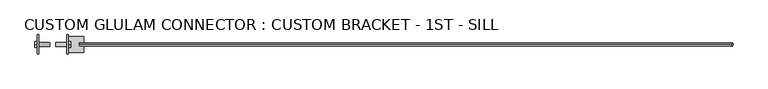
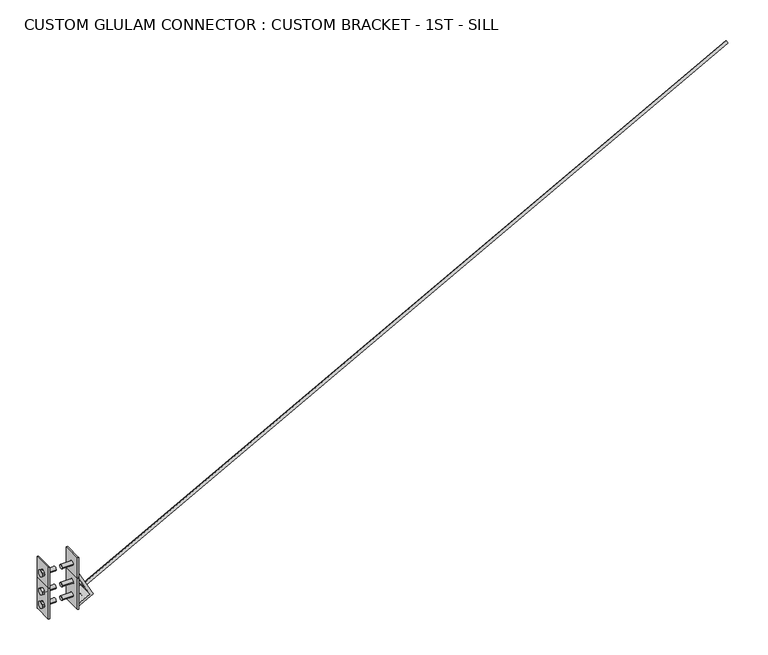
"""IFC4 building model written with IfcOpenShell, lengths in millimetres: fastener geometry, CUSTOM GLULAM CONNECTOR : CUSTOM BRACKET - 1ST - SILL."""

from ifc_helpers import new_model, si_unit, point, frame, frame_2d, origin, place, context, project, spatial, polyline, circle_curve, trimmed, segment, composite_curve, outline, extrude, source, transform, mapped, element, save
from ifc_brep_helpers import plane_surface, revolved_surface, advanced_brep


def custom_glulam_connector_custom_bracket_1st_sill_b9bb6f32(model_context):
    return source(origin(), model_context, "Body", "SolidModel", [
        advanced_brep(
        [(-87.3125, -13.890625, 160.3375), (-87.3125, 13.890625, 160.3375), (-95.25, 13.890625, 160.3375), (-95.25, -13.890625, 160.3375), (-95.25, 60.325, 211.1375), (-95.25, 60.325, 7.9375), (-95.25, 52.3875, 7.9375), (-95.25, -60.325, 7.9375), (-95.25, -60.325, 211.1375), (-95.25, 52.3875, 211.1375), (-95.25, 13.890625, 71.4375), (-95.25, -13.890625, 71.4375), (-87.3125, 13.890625, 71.4375), (-87.3125, -13.890625, 71.4375), (-87.3125, 60.325, 211.1375), (-87.3125, -60.325, 211.1375), (-87.3125, -60.325, 7.9375), (-87.3125, 60.325, 7.9375)],
        [
            (0, 1, circle_curve(frame((-87.3125, 0.0, 160.3375), z_axis=(1.0, 0.0, 0.0), x_axis=(0.0, 1.0, 0.0)), 13.890625)),
            (1, 2),
            (2, 3, circle_curve(frame((-95.25, 0.0, 160.3375), z_axis=(-1.0, 0.0, 0.0), x_axis=(0.0, 1.0, 0.0)), 13.890625)),
            (3, 0),
            (4, 5),
            (5, 6),
            (6, 7),
            (7, 8),
            (8, 9),
            (9, 4),
            (10, 11, circle_curve(frame((-95.25, 0.0, 71.4375), z_axis=(1.0, 0.0, 0.0), x_axis=(0.0, 1.0, 0.0)), 13.890625)),
            (11, 10, circle_curve(frame((-95.25, 0.0, 71.4375), z_axis=(1.0, 0.0, 0.0), x_axis=(0.0, 1.0, 0.0)), 13.890625)),
            (2, 3, circle_curve(frame((-95.25, 0.0, 160.3375), z_axis=(1.0, 0.0, 0.0), x_axis=(0.0, 1.0, 0.0)), 13.890625)),
            (10, 12),
            (12, 13, circle_curve(frame((-87.3125, 0.0, 71.4375), z_axis=(1.0, 0.0, 0.0), x_axis=(0.0, 1.0, 0.0)), 13.890625)),
            (13, 11),
            (1, 0, circle_curve(frame((-87.3125, 0.0, 160.3375), z_axis=(1.0, 0.0, 0.0), x_axis=(0.0, 1.0, 0.0)), 13.890625)),
            (13, 12, circle_curve(frame((-87.3125, 0.0, 71.4375), z_axis=(1.0, 0.0, 0.0), x_axis=(0.0, 1.0, 0.0)), 13.890625)),
            (14, 15),
            (15, 16),
            (16, 17),
            (17, 14),
            (8, 15),
            (14, 4),
            (7, 16),
            (5, 17),
        ],
        [
            revolved_surface(polyline([(-95.25, 13.890625, 160.3375), (-87.3125, 13.890625, 160.3375)]), (-87.3125, 0.0, 160.3375), (-1.0, 0.0, 0.0)),
            plane_surface(frame((-95.25, -60.325, 211.1375), z_axis=(-1.0, 0.0, 0.0), x_axis=(0.0, -1.0, 0.0))),
            revolved_surface(polyline([(-95.25, 13.890625, 71.4375), (-87.3125, 13.890625, 71.4375)]), (-87.3125, 0.0, 71.4375), (-1.0, 0.0, 0.0)),
            plane_surface(frame((-87.3125, -60.325, 211.1375), z_axis=(1.0, 0.0, 0.0), x_axis=(0.0, 1.0, 0.0))),
            plane_surface(frame((-95.25, 60.325, 211.1375), z_axis=(0.0, 0.0, 1.0), x_axis=(1.0, 0.0, 0.0))),
            plane_surface(frame((-95.25, -60.325, 211.1375), z_axis=(0.0, -1.0, 0.0), x_axis=(1.0, 0.0, 0.0))),
            plane_surface(frame((-95.25, -60.325, 7.9375), z_axis=(0.0, 0.0, -1.0), x_axis=(1.0, 0.0, 0.0))),
            plane_surface(frame((-95.25, 60.325, 7.9375), z_axis=(0.0, 1.0, 0.0), x_axis=(1.0, 0.0, 0.0))),
        ],
        [
            (0, [[1, 2, 3, 4]]),
            (1, [[5, 6, 7, 8, 9, 10], [11, 12], [13, -3]]),
            (2, [[-11, 14, 15, 16]]),
            (0, [[-13, -2, 17, -4]]),
            (2, [[18, -14, -12, -16]]),
            (3, [[19, 20, 21, 22], [-17, -1], [-15, -18]]),
            (4, [[23, -19, 24, -10, -9]]),
            (5, [[25, -20, -23, -8]]),
            (6, [[26, -21, -25, -7, -6]]),
            (7, [[-24, -22, -26, -5]]),
        ],
    ),
        extrude(outline(polyline([(-19.05, 171.3360226), (0.0, 182.3345453), (19.05, 171.3360226), (19.05, 149.3389774), (0.0, 138.3404547), (-19.05, 149.3389774), (-19.05, 171.3360226)])), frame((-110.2320312, 0.0, 0.0), z_axis=(1.0, 0.0, 0.0), x_axis=(0.0, 1.0, 0.0)), (0.0, 0.0, 1.0), 14.9820312),
        extrude(outline(composite_curve([segment(trimmed(circle_curve(frame_2d((0.0, 160.3375)), 12.7), [point((-12.7, 160.3375))], [point((12.7, 160.3375))], False, "CARTESIAN"), True, "CONTINUOUS"), segment(trimmed(circle_curve(frame_2d((0.0, 160.3375)), 12.7), [point((12.7, 160.3375))], [point((-12.7, 160.3375))], False, "CARTESIAN"), True, "CONTINUOUS")], self_intersect=False)), frame((-95.25, 0.0, 0.0), z_axis=(1.0, 0.0, 0.0), x_axis=(0.0, 1.0, 0.0)), (0.0, 0.0, 1.0), 76.2),
        extrude(outline(polyline([(-19.05, 82.4360226), (0.0, 93.4345453), (19.05, 82.4360226), (19.05, 60.4389774), (0.0, 49.4404547), (-19.05, 60.4389774), (-19.05, 82.4360226)])), frame((-110.2320312, 0.0, 0.0), z_axis=(1.0, 0.0, 0.0), x_axis=(0.0, 1.0, 0.0)), (0.0, 0.0, 1.0), 14.9820312),
        extrude(outline(composite_curve([segment(trimmed(circle_curve(frame_2d((0.0, 71.4375)), 12.7), [point((-12.7, 71.4375))], [point((12.7, 71.4375))], False, "CARTESIAN"), True, "CONTINUOUS"), segment(trimmed(circle_curve(frame_2d((0.0, 71.4375)), 12.7), [point((12.7, 71.4375))], [point((-12.7, 71.4375))], False, "CARTESIAN"), True, "CONTINUOUS")], self_intersect=False)), frame((-95.25, 0.0, 0.0), z_axis=(1.0, 0.0, 0.0), x_axis=(0.0, 1.0, 0.0)), (0.0, 0.0, 1.0), 76.2),
        extrude(outline(polyline([(-19.05, 171.3360226), (0.0, 182.3345453), (19.05, 171.3360226), (19.05, 149.3389774), (0.0, 138.3404547), (-19.05, 149.3389774), (-19.05, 171.3360226)])), frame((-110.2320312, 0.0, 0.0), z_axis=(1.0, 0.0, 0.0), x_axis=(0.0, 1.0, 0.0)), (0.0, 0.0, 1.0), 14.9820312),
        extrude(outline(composite_curve([segment(trimmed(circle_curve(frame_2d((0.0, 160.3375)), 12.7), [point((-12.7, 160.3375))], [point((12.7, 160.3375))], False, "CARTESIAN"), True, "CONTINUOUS"), segment(trimmed(circle_curve(frame_2d((0.0, 160.3375)), 12.7), [point((12.7, 160.3375))], [point((-12.7, 160.3375))], False, "CARTESIAN"), True, "CONTINUOUS")], self_intersect=False)), frame((-95.25, 0.0, 0.0), z_axis=(1.0, 0.0, 0.0), x_axis=(0.0, 1.0, 0.0)), (0.0, 0.0, 1.0), 76.2),
        extrude(outline(polyline([(-19.05, 171.3360226), (0.0, 182.3345453), (19.05, 171.3360226), (19.05, 149.3389774), (0.0, 138.3404547), (-19.05, 149.3389774), (-19.05, 171.3360226)])), frame((95.25, 0.0, 0.0), z_axis=(1.0, 0.0, 0.0), x_axis=(0.0, 1.0, 0.0)), (0.0, 0.0, 1.0), 14.9820312),
        extrude(outline(composite_curve([segment(trimmed(circle_curve(frame_2d((0.0, 160.3375)), 12.7), [point((-12.7, 160.3375))], [point((12.7, 160.3375))], False, "CARTESIAN"), True, "CONTINUOUS"), segment(trimmed(circle_curve(frame_2d((0.0, 160.3375)), 12.7), [point((12.7, 160.3375))], [point((-12.7, 160.3375))], False, "CARTESIAN"), True, "CONTINUOUS")], self_intersect=False)), frame((19.05, 0.0, 0.0), z_axis=(1.0, 0.0, 0.0), x_axis=(0.0, 1.0, 0.0)), (0.0, 0.0, 1.0), 76.2),
        extrude(outline(polyline([(-19.05, 82.4360226), (0.0, 93.4345453), (19.05, 82.4360226), (19.05, 60.4389774), (0.0, 49.4404547), (-19.05, 60.4389774), (-19.05, 82.4360226)])), frame((95.25, 0.0, 0.0), z_axis=(1.0, 0.0, 0.0), x_axis=(0.0, 1.0, 0.0)), (0.0, 0.0, 1.0), 14.9820312),
        extrude(outline(composite_curve([segment(trimmed(circle_curve(frame_2d((0.0, 71.4375)), 12.7), [point((-12.7, 71.4375))], [point((12.7, 71.4375))], False, "CARTESIAN"), True, "CONTINUOUS"), segment(trimmed(circle_curve(frame_2d((0.0, 71.4375)), 12.7), [point((12.7, 71.4375))], [point((-12.7, 71.4375))], False, "CARTESIAN"), True, "CONTINUOUS")], self_intersect=False)), frame((19.05, 0.0, 0.0), z_axis=(1.0, 0.0, 0.0), x_axis=(0.0, 1.0, 0.0)), (0.0, 0.0, 1.0), 76.2),
        extrude(outline(polyline([(-19.05, 171.3360226), (0.0, 182.3345453), (19.05, 171.3360226), (19.05, 149.3389774), (0.0, 138.3404547), (-19.05, 149.3389774), (-19.05, 171.3360226)])), frame((95.25, 0.0, 0.0), z_axis=(1.0, 0.0, 0.0), x_axis=(0.0, 1.0, 0.0)), (0.0, 0.0, 1.0), 14.9820312),
        extrude(outline(composite_curve([segment(trimmed(circle_curve(frame_2d((0.0, 160.3375)), 12.7), [point((-12.7, 160.3375))], [point((12.7, 160.3375))], False, "CARTESIAN"), True, "CONTINUOUS"), segment(trimmed(circle_curve(frame_2d((0.0, 160.3375)), 12.7), [point((12.7, 160.3375))], [point((-12.7, 160.3375))], False, "CARTESIAN"), True, "CONTINUOUS")], self_intersect=False)), frame((19.05, 0.0, 0.0), z_axis=(1.0, 0.0, 0.0), x_axis=(0.0, 1.0, 0.0)), (0.0, 0.0, 1.0), 76.2),
        advanced_brep(
        [(87.3125, -13.890625, 160.3375), (95.25, -13.890625, 160.3375), (95.25, 13.890625, 160.3375), (87.3125, 13.890625, 160.3375), (95.25, 60.325, 211.1375), (95.25, 52.3875, 211.1375), (95.25, -60.325, 211.1375), (95.25, -60.325, 7.9375), (95.25, 52.3875, 7.9375), (95.25, 60.325, 7.9375), (95.25, 13.890625, 71.4375), (95.25, -13.890625, 71.4375), (87.3125, -13.890625, 71.4375), (87.3125, 13.890625, 71.4375), (87.3125, 60.325, 211.1375), (87.3125, 60.325, 7.9375), (87.3125, -60.325, 7.9375), (87.3125, -60.325, 211.1375)],
        [
            (0, 1),
            (1, 2, circle_curve(frame((95.25, 0.0, 160.3375), z_axis=(1.0, 0.0, 0.0), x_axis=(0.0, 1.0, 0.0)), 13.890625)),
            (2, 3),
            (3, 0, circle_curve(frame((87.3125, 0.0, 160.3375), z_axis=(-1.0, 0.0, 0.0), x_axis=(0.0, 1.0, 0.0)), 13.890625)),
            (4, 5),
            (5, 6),
            (6, 7),
            (7, 8),
            (8, 9),
            (9, 4),
            (1, 2, circle_curve(frame((95.25, 0.0, 160.3375), z_axis=(-1.0, 0.0, 0.0), x_axis=(0.0, 1.0, 0.0)), 13.890625)),
            (10, 11, circle_curve(frame((95.25, 0.0, 71.4375), z_axis=(-1.0, 0.0, 0.0), x_axis=(0.0, 1.0, 0.0)), 13.890625)),
            (11, 10, circle_curve(frame((95.25, 0.0, 71.4375), z_axis=(-1.0, 0.0, 0.0), x_axis=(0.0, 1.0, 0.0)), 13.890625)),
            (11, 12),
            (12, 13, circle_curve(frame((87.3125, 0.0, 71.4375), z_axis=(-1.0, 0.0, 0.0), x_axis=(0.0, 1.0, 0.0)), 13.890625)),
            (13, 10),
            (0, 3, circle_curve(frame((87.3125, 0.0, 160.3375), z_axis=(-1.0, 0.0, 0.0), x_axis=(0.0, 1.0, 0.0)), 13.890625)),
            (13, 12, circle_curve(frame((87.3125, 0.0, 71.4375), z_axis=(-1.0, 0.0, 0.0), x_axis=(0.0, 1.0, 0.0)), 13.890625)),
            (14, 15),
            (15, 16),
            (16, 17),
            (17, 14),
            (4, 14),
            (17, 6),
            (16, 7),
            (15, 9),
        ],
        [
            revolved_surface(polyline([(95.25, 13.890625, 160.3375), (87.3125, 13.890625, 160.3375)]), (87.3125, 0.0, 160.3375), (1.0, 0.0, 0.0)),
            plane_surface(frame((95.25, -60.325, 211.1375), z_axis=(1.0, 0.0, 0.0), x_axis=(0.0, -1.0, 0.0))),
            revolved_surface(polyline([(95.25, 13.890625, 71.4375), (87.3125, 13.890625, 71.4375)]), (87.3125, 0.0, 71.4375), (1.0, 0.0, 0.0)),
            plane_surface(frame((87.3125, -60.325, 211.1375), z_axis=(-1.0, 0.0, 0.0), x_axis=(0.0, 1.0, 0.0))),
            plane_surface(frame((95.25, 60.325, 211.1375), z_axis=(0.0, 0.0, 1.0), x_axis=(-1.0, 0.0, 0.0))),
            plane_surface(frame((95.25, -60.325, 211.1375), z_axis=(0.0, -1.0, 0.0), x_axis=(-1.0, 0.0, 0.0))),
            plane_surface(frame((95.25, -60.325, 7.9375), z_axis=(0.0, 0.0, -1.0), x_axis=(-1.0, 0.0, 0.0))),
            plane_surface(frame((95.25, 60.325, 7.9375), z_axis=(0.0, 1.0, 0.0), x_axis=(-1.0, 0.0, 0.0))),
        ],
        [
            (0, [[1, 2, 3, 4]]),
            (1, [[5, 6, 7, 8, 9, 10], [-2, 11], [12, 13]]),
            (2, [[14, 15, 16, -13]]),
            (0, [[-1, 17, -3, -11]]),
            (2, [[-14, -12, -16, 18]]),
            (3, [[19, 20, 21, 22], [-4, -17], [-18, -15]]),
            (4, [[-6, -5, 23, -22, 24]]),
            (5, [[-7, -24, -21, 25]]),
            (6, [[-9, -8, -25, -20, 26]]),
            (7, [[-10, -26, -19, -23]]),
        ],
    ),
        extrude(outline(polyline([(-19.05, 291.9860226), (0.0, 302.9845453), (19.05, 291.9860226), (19.05, 269.9889774), (0.0, 258.9904547), (-19.05, 269.9889774), (-19.05, 291.9860226)])), frame((-110.2320312, 0.0, 0.0), z_axis=(1.0, 0.0, 0.0), x_axis=(0.0, 1.0, 0.0)), (0.0, 0.0, 1.0), 14.9820312),
        extrude(outline(composite_curve([segment(trimmed(circle_curve(frame_2d((0.0, 280.9875)), 12.7), [point((-12.7, 280.9875))], [point((12.7, 280.9875))], False, "CARTESIAN"), True, "CONTINUOUS"), segment(trimmed(circle_curve(frame_2d((0.0, 280.9875)), 12.7), [point((12.7, 280.9875))], [point((-12.7, 280.9875))], False, "CARTESIAN"), True, "CONTINUOUS")], self_intersect=False)), frame((-95.25, 0.0, 0.0), z_axis=(1.0, 0.0, 0.0), x_axis=(0.0, 1.0, 0.0)), (0.0, 0.0, 1.0), 76.2),
        advanced_brep(
        [(-95.25, 60.325, 350.8375), (-87.3125, 60.325, 350.8375), (-87.3125, 60.325, 211.1375), (-95.25, 60.325, 211.1375), (-87.3125, -13.890625, 280.9875), (-87.3125, 13.890625, 280.9875), (-95.25, 13.890625, 280.9875), (-95.25, -13.890625, 280.9875), (-95.25, -60.325, 350.8375), (-87.3125, -60.325, 350.8375), (-95.25, -52.3875, 350.8375), (-95.25, -52.3875, 211.1375), (-95.25, -60.325, 211.1375), (-87.3125, -60.325, 211.1375)],
        [
            (0, 1),
            (1, 2),
            (2, 3),
            (3, 0),
            (4, 5, circle_curve(frame((-87.3125, 0.0, 280.9875), z_axis=(1.0, 0.0, 0.0), x_axis=(0.0, 1.0, 0.0)), 13.890625)),
            (5, 6),
            (6, 7, circle_curve(frame((-95.25, 0.0, 280.9875), z_axis=(-1.0, 0.0, 0.0), x_axis=(0.0, 1.0, 0.0)), 13.890625)),
            (7, 4),
            (7, 6, circle_curve(frame((-95.25, 0.0, 280.9875), z_axis=(-1.0, 0.0, 0.0), x_axis=(0.0, 1.0, 0.0)), 13.890625)),
            (5, 4, circle_curve(frame((-87.3125, 0.0, 280.9875), z_axis=(1.0, 0.0, 0.0), x_axis=(0.0, 1.0, 0.0)), 13.890625)),
            (8, 9),
            (9, 1),
            (0, 10),
            (10, 8),
            (3, 11),
            (11, 12),
            (12, 8),
            (9, 13),
            (13, 2),
            (12, 13),
        ],
        [
            plane_surface(frame((-95.25, 60.325, 211.1375), z_axis=(0.0, 1.0, 0.0), x_axis=(1.0, 0.0, 0.0))),
            revolved_surface(polyline([(-95.25, 13.890625, 280.9875), (-87.3125, 13.890625, 280.9875)]), (-87.3125, 0.0, 280.9875), (-1.0, 0.0, 0.0)),
            plane_surface(frame((-95.25, 60.325, 350.8375), z_axis=(0.0, 0.0, 1.0), x_axis=(1.0, 0.0, 0.0))),
            plane_surface(frame((-95.25, -60.325, 350.8375), z_axis=(-1.0, 0.0, 0.0), x_axis=(0.0, -1.0, 0.0))),
            plane_surface(frame((-87.3125, -60.325, 350.8375), z_axis=(1.0, 0.0, 0.0), x_axis=(0.0, 1.0, 0.0))),
            plane_surface(frame((-95.25, -60.325, 350.8375), z_axis=(0.0, -1.0, 0.0), x_axis=(1.0, 0.0, 0.0))),
            plane_surface(frame((-95.25, -60.325, 211.1375), z_axis=(0.0, 0.0, -1.0), x_axis=(1.0, 0.0, 0.0))),
        ],
        [
            (0, [[1, 2, 3, 4]]),
            (1, [[5, 6, 7, 8]]),
            (1, [[9, -6, 10, -8]]),
            (2, [[11, 12, -1, 13, 14]]),
            (3, [[-4, 15, 16, 17, -14, -13], [-9, -7]]),
            (4, [[-12, 18, 19, -2], [-10, -5]]),
            (5, [[20, -18, -11, -17]]),
            (6, [[-3, -19, -20, -16, -15]]),
        ],
    ),
        advanced_brep(
        [(95.25, 60.325, 350.8375), (95.25, 60.325, 211.1375), (87.3125, 60.325, 211.1375), (87.3125, 60.325, 350.8375), (87.3125, -13.890625, 280.9875), (95.25, -13.890625, 280.9875), (95.25, 13.890625, 280.9875), (87.3125, 13.890625, 280.9875), (95.25, -60.325, 350.8375), (95.25, -52.3875, 350.8375), (87.3125, -60.325, 350.8375), (95.25, -60.325, 211.1375), (95.25, -52.3875, 211.1375), (87.3125, -60.325, 211.1375)],
        [
            (0, 1),
            (1, 2),
            (2, 3),
            (3, 0),
            (4, 5),
            (5, 6, circle_curve(frame((95.25, 0.0, 280.9875), z_axis=(1.0, 0.0, 0.0), x_axis=(0.0, 1.0, 0.0)), 13.890625)),
            (6, 7),
            (7, 4, circle_curve(frame((87.3125, 0.0, 280.9875), z_axis=(-1.0, 0.0, 0.0), x_axis=(0.0, 1.0, 0.0)), 13.890625)),
            (4, 7, circle_curve(frame((87.3125, 0.0, 280.9875), z_axis=(-1.0, 0.0, 0.0), x_axis=(0.0, 1.0, 0.0)), 13.890625)),
            (6, 5, circle_curve(frame((95.25, 0.0, 280.9875), z_axis=(1.0, 0.0, 0.0), x_axis=(0.0, 1.0, 0.0)), 13.890625)),
            (8, 9),
            (9, 0),
            (3, 10),
            (10, 8),
            (8, 11),
            (11, 12),
            (12, 1),
            (2, 13),
            (13, 10),
            (13, 11),
        ],
        [
            plane_surface(frame((95.25, 60.325, 211.1375), z_axis=(0.0, 1.0, 0.0), x_axis=(-1.0, 0.0, 0.0))),
            revolved_surface(polyline([(95.25, 13.890625, 280.9875), (87.3125, 13.890625, 280.9875)]), (87.3125, 0.0, 280.9875), (1.0, 0.0, 0.0)),
            plane_surface(frame((95.25, 60.325, 350.8375), z_axis=(0.0, 0.0, 1.0), x_axis=(-1.0, 0.0, 0.0))),
            plane_surface(frame((95.25, -60.325, 350.8375), z_axis=(1.0, 0.0, 0.0), x_axis=(0.0, -1.0, 0.0))),
            plane_surface(frame((87.3125, -60.325, 350.8375), z_axis=(-1.0, 0.0, 0.0), x_axis=(0.0, 1.0, 0.0))),
            plane_surface(frame((95.25, -60.325, 350.8375), z_axis=(0.0, -1.0, 0.0), x_axis=(-1.0, 0.0, 0.0))),
            plane_surface(frame((95.25, -60.325, 211.1375), z_axis=(0.0, 0.0, -1.0), x_axis=(-1.0, 0.0, 0.0))),
        ],
        [
            (0, [[1, 2, 3, 4]]),
            (1, [[5, 6, 7, 8]]),
            (1, [[-5, 9, -7, 10]]),
            (2, [[11, 12, -4, 13, 14]]),
            (3, [[-12, -11, 15, 16, 17, -1], [-6, -10]]),
            (4, [[-3, 18, 19, -13], [-8, -9]]),
            (5, [[-15, -14, -19, 20]]),
            (6, [[-17, -16, -20, -18, -2]]),
        ],
    ),
        extrude(outline(polyline([(-19.05, 291.9860226), (0.0, 302.9845453), (19.05, 291.9860226), (19.05, 269.9889774), (0.0, 258.9904547), (-19.05, 269.9889774), (-19.05, 291.9860226)])), frame((95.25, 0.0, 0.0), z_axis=(1.0, 0.0, 0.0), x_axis=(0.0, 1.0, 0.0)), (0.0, 0.0, 1.0), 14.9820312),
        extrude(outline(composite_curve([segment(trimmed(circle_curve(frame_2d((0.0, 280.9875)), 12.7), [point((-12.7, 280.9875))], [point((12.7, 280.9875))], False, "CARTESIAN"), True, "CONTINUOUS"), segment(trimmed(circle_curve(frame_2d((0.0, 280.9875)), 12.7), [point((12.7, 280.9875))], [point((-12.7, 280.9875))], False, "CARTESIAN"), True, "CONTINUOUS")], self_intersect=False)), frame((19.05, 0.0, 0.0), z_axis=(1.0, 0.0, 0.0), x_axis=(0.0, 1.0, 0.0)), (0.0, 0.0, 1.0), 76.2),
        extrude(outline(composite_curve([segment(trimmed(circle_curve(frame_2d((0.0, -9.525)), 9.525), [point((0.0, -19.05))], [point((0.0, 0.0))], False, "CARTESIAN"), True, "CONTINUOUS"), segment(trimmed(circle_curve(frame_2d((0.0, -9.525)), 9.525), [point((0.0, 0.0))], [point((0.0, -19.05))], False, "CARTESIAN"), True, "CONTINUOUS")], self_intersect=False)), frame((173.2138238, 0.0, 105.1724436), z_axis=(0.8788171126619665, 0.0, 0.4771587602596065), x_axis=(0.0, -1.0, 0.0)), (0.0, 0.0, 1.0), 4597.4),
        advanced_brep(
        [(192.9085516, -50.8, 68.8992672), (95.25, -50.8, 248.7639444), (95.25, -50.8, 215.4940952), (171.3824347, -50.8, 75.2755936), (95.25, -50.8, 33.9390543), (95.25, -50.8, 15.875), (192.9085516, 50.8, 68.8992672), (95.25, 50.8, 15.875), (95.25, 50.8, 33.9390543), (171.3824347, 50.8, 75.2755936), (95.25, 50.8, 215.4940952), (95.25, 50.8, 248.7639444), (173.781941, 0.0, 104.1261019), (163.5558323, 0.0, 122.9602512), (149.6046106, 0.0, 115.3853559), (159.8307193, 0.0, 96.5512066), (141.0385275, 0.0, 58.8001963), (140.3409665, 0.0, 58.4214515), (147.9158618, 0.0, 44.4702298), (148.6134229, 0.0, 44.8489746)],
        [
            (0, 1),
            (1, 2),
            (2, 3),
            (3, 4),
            (4, 5),
            (5, 0),
            (6, 7),
            (7, 8),
            (8, 9),
            (9, 10),
            (10, 11),
            (11, 6),
            (0, 6),
            (11, 1),
            (12, 13, circle_curve(frame((168.6688866, 0.0, 113.5431766), z_axis=(-0.8788171126619665, 0.0, -0.4771587602596065), x_axis=(-0.4771587602596065, 0.0, 0.8788171126619665)), 10.715625)),
            (13, 12, circle_curve(frame((168.6688866, 0.0, 113.5431766), z_axis=(-0.8788171126619665, 0.0, -0.4771587602596065), x_axis=(-0.4771587602596065, 0.0, 0.8788171126619665)), 10.715625)),
            (10, 2),
            (9, 3),
            (14, 15, circle_curve(frame((154.717665, 0.0, 105.9682812), z_axis=(0.8788171126619665, 0.0, 0.4771587602596065), x_axis=(-0.4771587602596065, 0.0, 0.8788171126619665)), 10.715625)),
            (15, 14, circle_curve(frame((154.717665, 0.0, 105.9682812), z_axis=(0.8788171126619665, 0.0, 0.4771587602596065), x_axis=(-0.4771587602596065, 0.0, 0.8788171126619665)), 10.715625)),
            (8, 4),
            (16, 17, circle_curve(frame((140.689747, 0.0, 58.6108239), z_axis=(0.47715876025960524, 0.0, -0.8788171126619673), x_axis=(0.878817112661967, 0.0, 0.47715876025960513)), 0.396875)),
            (17, 16, circle_curve(frame((140.689747, 0.0, 58.6108239), z_axis=(0.47715876025960524, 0.0, -0.8788171126619673), x_axis=(0.878817112661967, 0.0, 0.47715876025960513)), 0.396875)),
            (7, 5),
            (18, 19, circle_curve(frame((148.2646423, 0.0, 44.6596022), z_axis=(-0.47715876025960524, 0.0, 0.8788171126619673), x_axis=(0.878817112661967, 0.0, 0.47715876025960513)), 0.396875)),
            (19, 18, circle_curve(frame((148.2646423, 0.0, 44.6596022), z_axis=(-0.47715876025960524, 0.0, 0.8788171126619673), x_axis=(0.878817112661967, 0.0, 0.47715876025960513)), 0.396875)),
            (12, 15),
            (14, 13),
            (18, 17),
            (16, 19),
        ],
        [
            plane_surface(frame((95.25, -50.8, 248.7639444), z_axis=(0.0, -1.0000000000000002, 0.0), x_axis=(-0.4771587602596065, 0.0, 0.8788171126619665))),
            plane_surface(frame((95.25, 50.8, 248.7639444), z_axis=(0.0, 1.0000000000000002, 0.0), x_axis=(0.4771587602596065, 0.0, -0.8788171126619665))),
            plane_surface(frame((192.9085516, -50.8, 68.8992672), z_axis=(0.8788171126619665, 0.0, 0.4771587602596065), x_axis=(0.0, 1.0, 0.0))),
            plane_surface(frame((95.25, -50.8, 248.7639444), z_axis=(-1.0, 0.0, 0.0), x_axis=(0.0, 1.0, 0.0))),
            plane_surface(frame((95.25, -50.8, 215.4940952), z_axis=(-0.8788171126619664, 0.0, -0.4771587602596066), x_axis=(0.0, 1.0, 0.0))),
            plane_surface(frame((171.3824347, -50.8, 75.2755936), z_axis=(-0.4771587602596049, 0.0, 0.8788171126619674), x_axis=(0.0, 1.0, 0.0))),
            plane_surface(frame((95.25, -50.8, 33.9390543), z_axis=(-1.0, 0.0, 0.0), x_axis=(0.0, 1.0, 0.0))),
            plane_surface(frame((95.25, -50.8, 15.875), z_axis=(0.4771587602596052, 0.0, -0.8788171126619672), x_axis=(0.0, 1.0, 0.0))),
            revolved_surface(polyline([(149.60461058960067, 0.0, 115.38535590022673), (163.55583228121063, 0.0, 122.9602512346057)]), (168.6688866, 0.0, 113.5431766), (-0.8788171126619665, 0.0, -0.4771587602596065)),
            revolved_surface(polyline([(141.0385274949113, 0.0, 58.80019629723707), (148.61342285819435, 0.0, 44.848974552392434)]), (148.2646423, 0.0, 44.6596022), (-0.47715876025960513, 0.0, 0.878817112661967)),
        ],
        [
            (0, [[1, 2, 3, 4, 5, 6]]),
            (1, [[7, 8, 9, 10, 11, 12]]),
            (2, [[-1, 13, -12, 14], [15, 16]]),
            (3, [[-2, -14, -11, 17]]),
            (4, [[-3, -17, -10, 18], [19, 20]]),
            (5, [[-4, -18, -9, 21], [22, 23]]),
            (6, [[-5, -21, -8, 24]]),
            (7, [[-6, -24, -7, -13], [25, 26]]),
            (8, [[27, -19, 28, -15]]),
            (8, [[-27, -16, -28, -20]]),
            (9, [[29, -22, 30, -25]]),
            (9, [[-29, -26, -30, -23]]),
        ],
    ),
    ])


if __name__ == "__main__":
    model = new_model("IFC4")
    model_context = context("Model", 3, world=origin())
    ifc_project = project(units=[si_unit("LENGTHUNIT", "METRE", prefix="MILLI")], contexts=[model_context])
    site = spatial("IfcSite", under=ifc_project)
    building = spatial("IfcBuilding", under=site)
    placement = place(None, origin())
    custom_glulam_connector_custom_bracket_1st_sill_shape = custom_glulam_connector_custom_bracket_1st_sill_b9bb6f32(model_context)
    element("IfcFastener", 1, ObjectType="CUSTOM GLULAM CONNECTOR : CUSTOM BRACKET - 1ST - SILL", at=placement, inside=building, context=model_context, shape_type="MappedRepresentation", body=[
        mapped(custom_glulam_connector_custom_bracket_1st_sill_shape, transform((0.0, 0.0, 0.0), x_axis=(1.0, 0.0, 0.0), y_axis=(0.0, 1.0, 0.0), z_axis=(0.0, 0.0, 1.0))),
    ])
    save(model, "model.ifc")

# Revit data of these elements
# Type "CUSTOM GLULAM CONNECTOR : CUSTOM BRACKET - 1ST - SILL"
#   Width - Top = 0' - 6 7/8"
#   Top/Bottom Plate Thickness = 0' - 0 5/16"
#   Top/Bottom Plate - Width = 0' - 7 1/2"
#   Rod Radius = 0' - 0 3/8"
#   Rod Length [instance default] = 1' - 0"
#   Plate Thickness = 0' - 0 5/16"
#   Offset - Upper Plate 2 = 0' - 0"
#   Height of Plate = 0' - 8"
#   Width - Bottom = 0' - 6 7/8"
#   Plate Width = 0' - 4 3/4"
#   Bracket Width = 0' - 4"
#   Bracket Thickness = 0' - 0 5/8"
#   Bracket Offset in X = 0' - 3 3/4"
#   Bracket Offset in Y = 0' - 0 3/8"
#   Bracket Offset = 0' - 0 5/8"
#   Bracket Leg = 0' - 4 3/8"
#   Bracket Hole Radius - Up = 0' - 0 27/64"
#   Bracket Hole Radius - Down = 0' - 0 1/64"
#   Bracket Hole Offset = 0' - 2"
#   Beam Width = 0' - 7 3/8"
#   Angle 2 = 28.50°
#   Angle 1 = 118.50°
#   Top Plate Visible = no
#   Rod Visibility = yes
#   Plate Visibility - Upper Right 2 = no
#   Plate Visibility - Upper Right 1 = yes
#   Plate Visibility - Upper Left 2 = no
#   Plate Visibility - Upper Left 1 = yes
#   Plate Visibility - Lower Right 2 = no
#   Plate Visibility - Lower Right 1 = yes
#   Plate Visibility - Lower Left 2 = no
#   Plate Visibility - Lower Left 1 = yes
#   Bracket Visibility = yes
#   Bottom Plate Visible = no
#   Upper Plates - 2 = element 1323965
#   Upper Plates - 1 = element 1323965
#   Lower Plates = element 1339837
#   Bracket Material = 5/8" STEEL ANGLE (HDG AFTER FABRICATION)
#   URL = ""
# Element 1 (IfcFastener, "CUSTOM GLULAM CONNECTOR : CUSTOM BRACKET - 1ST - SILL")
#   Rod Length = 15' - 1"
#   Materials on its faces: "1\" GALV. LAG BOLT (LENGTH = 1/2\" SHY OF GLULAM DEPTH) -  (GALV. THRU BOLT IF PLATE ON OPP. SIDE OF STRUCT MEMBER)", "5/16\" STEEL PLATE (HDG AFTER FABRICATION)", "5/8\" STEEL ANGLE (HDG AFTER FABRICATION)", "3/4\" GALV. ROD (THREADED AT ENDS) - TURN BUCKLE AT 1/4 POINT OF TOTAL LENGTH"
# Materials
#   "5/8\" STEEL ANGLE (HDG AFTER FABRICATION)": class "Generic", colour RGB 195 195 195, transparency 0, Cost = 0
#   "1\" GALV. LAG BOLT (LENGTH = 1/2\" SHY OF GLULAM DEPTH) -  (GALV. THRU BOLT IF PLATE ON OPP. SIDE OF STRUCT MEMBER)": class "Generic", colour RGB 120 120 120, transparency 0, Cost = 0
#   "5/16\" STEEL PLATE (HDG AFTER FABRICATION)": class "Generic", colour RGB 232 232 232, transparency 0, Cost = 0
#   "3/4\" GALV. ROD (THREADED AT ENDS) - TURN BUCKLE AT 1/4 POINT OF TOTAL LENGTH": class "Generic", colour RGB 120 120 120, transparency 0, Cost = 0
